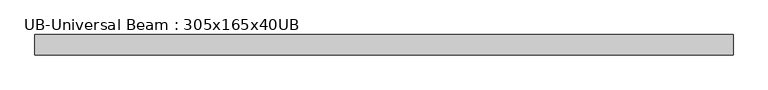
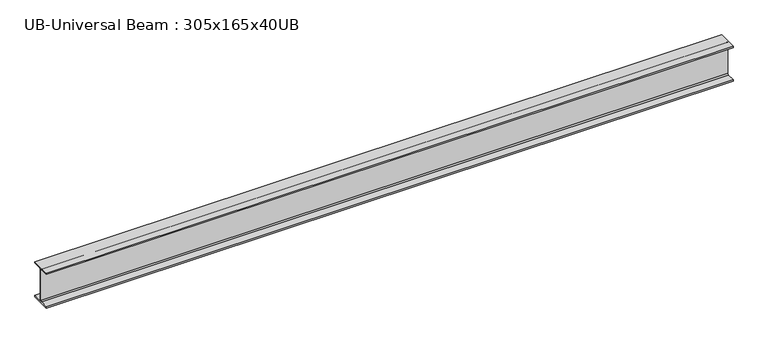
"""IFC4 building model written with IfcOpenShell, lengths in millimetres: beam geometry, UB-Universal Beam : 305x165x40UB."""

from ifc_helpers import new_model, si_unit, point, frame, frame_2d, origin, place, context, project, spatial, polyline, circle_curve, trimmed, segment, composite_curve, outline, extrude, source, transform, mapped, element, save


def ub_universal_beam_305x165x40ub_1ce0e142(model_context):
    return source(origin(), model_context, "Body", "SweptSolid", [
        extrude(outline(composite_curve([segment(polyline([(82.5, -141.5), (82.5, -151.7), (-82.5, -151.7), (-82.5, -141.5), (-11.9, -141.5)]), True, "CONTINUOUS"), segment(trimmed(circle_curve(frame_2d((-11.9, -132.6)), 8.9), [point((-11.9, -141.5))], [point((-3.0, -132.6))], True, "CARTESIAN"), True, "CONTINUOUS"), segment(polyline([(-3.0, -132.6), (-3.0, 132.6)]), True, "CONTINUOUS"), segment(trimmed(circle_curve(frame_2d((-11.9, 132.6)), 8.9), [point((-3.0, 132.6))], [point((-11.9, 141.5))], True, "CARTESIAN"), True, "CONTINUOUS"), segment(polyline([(-11.9, 141.5), (-82.5, 141.5), (-82.5, 151.7), (82.5, 151.7), (82.5, 141.5), (11.9, 141.5)]), True, "CONTINUOUS"), segment(trimmed(circle_curve(frame_2d((11.9, 132.6)), 8.9), [point((11.9, 141.5))], [point((3.0, 132.6))], True, "CARTESIAN"), True, "CONTINUOUS"), segment(polyline([(3.0, 132.6), (3.0, -132.6)]), True, "CONTINUOUS"), segment(trimmed(circle_curve(frame_2d((11.9, -132.6)), 8.9), [point((3.0, -132.6))], [point((11.9, -141.5))], True, "CARTESIAN"), True, "CONTINUOUS"), segment(polyline([(11.9, -141.5), (82.5, -141.5)]), True, "CONTINUOUS")], self_intersect=False)), frame((-2834.65, 0.0, 0.0), z_axis=(1.0, 0.0, 0.0), x_axis=(0.0, 1.0, 0.0)), (0.0, 0.0, 1.0), 5669.3),
    ])


if __name__ == "__main__":
    model = new_model("IFC4")
    model_context = context("Model", 3, world=origin())
    ifc_project = project(units=[si_unit("LENGTHUNIT", "METRE", prefix="MILLI")], contexts=[model_context])
    site = spatial("IfcSite", under=ifc_project)
    building = spatial("IfcBuilding", under=site)
    placement = place(None, origin())
    ub_universal_beam_305x165x40ub_shape = ub_universal_beam_305x165x40ub_1ce0e142(model_context)
    element("IfcBeam", 1, ObjectType="UB-Universal Beam : 305x165x40UB", at=placement, inside=building, context=model_context, shape_type="MappedRepresentation", body=[
        mapped(ub_universal_beam_305x165x40ub_shape, transform((0.0, 0.0, 0.0), x_axis=(1.0, 0.0, 0.0), y_axis=(0.0, 1.0, 0.0), z_axis=(0.0, 0.0, 1.0))),
    ])
    save(model, "model.ifc")

# Revit data of these elements
# Type "UB-Universal Beam : 305x165x40UB"
#   Nominal h = "305"
#   W = 0
#   Start Extension Calculation [instance default] = 3000 mm
#   Start Extension [instance default] = -12.7 mm
#   End Extension Calculation [instance default] = 3000 mm
#   End Extension [instance default] = -12.7 mm
#   Ix = 8503
#   Length [instance default] = 1524 mm
#   M = 40.3
#   Zx = 560
#   b = 165 mm
#   h = 303.4 mm
#   r = 8.9 mm
#   s = 6 mm
#   t = 10.2 mm
#   A = 0.005 m²
#   Structural Material [instance default] = Metal - Steel - 345 MPa
#   Assembly Code = ""
# Element 1 (IfcBeam, "UB-Universal Beam : 305x165x40UB")
#   Materials on its faces: "Metal - Steel - 345 MPa"
# Materials
#   "Metal - Steel - 345 MPa": class "Metal", colour RGB 241 46 46, transparency 0
